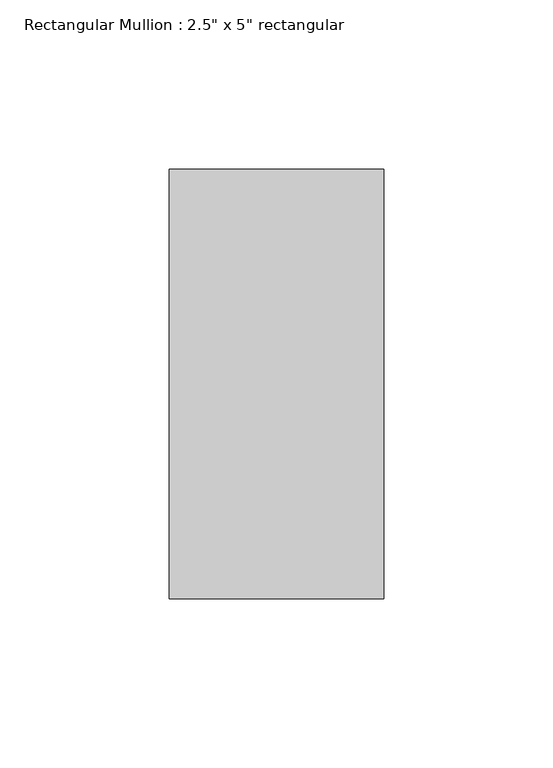
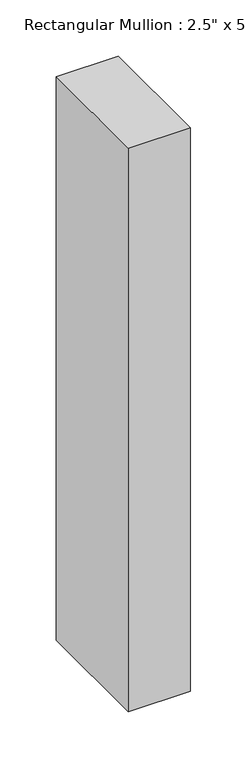
"""IFC4 building model written with IfcOpenShell, lengths in millimetres: member geometry."""

import ifcopenshell
import ifcopenshell.guid

model = None  # the IFC model being written
_history = None  # IfcOwnerHistory: only IFC2X3 demands one
_inside = {}  # id of a spatial element -> (the spatial element, [elements in it])
_under = {}  # id of a project, library or spatial element -> (it, [spatial elements below it])
_declared = {}  # id of a project -> (the project, [libraries it declares])
_typed = {}  # id of a type object -> (the type object, [elements of that type])
_made_of = {}  # id of a material, layer set ... -> (it, [elements and type objects made of it])


def new_model(schema):
    """Start an empty IFC model of exactly this schema.

    Asked for "IFC4X3", IfcOpenShell would pick the latest addendum, in which some entities
    have other attributes; the version numbers below select the first issue.
    IFC2X3 requires an IfcOwnerHistory on every rooted entity: one is made here for all.
    """
    global model, _history
    if schema == "IFC4X3":
        model = ifcopenshell.file(schema_version=(4, 3, 0, 0))
    else:
        model = ifcopenshell.file(schema=schema)
    _inside.clear()
    _under.clear()
    _declared.clear()
    _typed.clear()
    _made_of.clear()
    _history = None
    if model.schema == "IFC2X3":
        org = make("IfcOrganization", Name="unknown")
        user = make(
            "IfcPersonAndOrganization",
            ThePerson=make("IfcPerson", FamilyName="unknown"),
            TheOrganization=org,
        )
        app = make(
            "IfcApplication",
            ApplicationDeveloper=org,
            Version="unknown",
            ApplicationFullName="unknown",
            ApplicationIdentifier="unknown",
        )
        _history = make(
            "IfcOwnerHistory",
            OwningUser=user,
            OwningApplication=app,
            ChangeAction="ADDED",
            CreationDate=0,
        )
    return model


def make(cls, **values):
    """One entity of the class cls with the attributes given. An attribute that is None is left unset."""
    return model.create_entity(
        cls, **{name: value for name, value in values.items() if value is not None}
    )


def rooted(cls, **values):
    """An entity with a GlobalId (a new one), such as an element, a storey or a relation."""
    return make(cls, GlobalId=ifcopenshell.guid.new(), OwnerHistory=_history, **values)


def si_unit(unit_type, name, prefix=None):
    """IfcSIUnit, for example si_unit("LENGTHUNIT", "METRE", prefix="MILLI")."""
    return make("IfcSIUnit", UnitType=unit_type, Prefix=prefix, Name=name)


def assignment(units):
    """IfcUnitAssignment: the units of a project."""
    return None if units is None else make("IfcUnitAssignment", Units=units)


def point(xyz):
    """IfcCartesianPoint."""
    return None if xyz is None else make("IfcCartesianPoint", Coordinates=xyz)


def direction(xyz):
    """IfcDirection."""
    return None if xyz is None else make("IfcDirection", DirectionRatios=xyz)


def frame(location, z_axis=None, x_axis=None):
    """IfcAxis2Placement3D, a coordinate frame: its origin and axes. An axis left out is left unset."""
    return make(
        "IfcAxis2Placement3D",
        Location=point(location),
        Axis=direction(z_axis),
        RefDirection=direction(x_axis),
    )


def origin():
    """The frame at (0, 0, 0) with its axes left unset."""
    return frame((0.0, 0.0, 0.0))


def place(relative_to, where):
    """IfcLocalPlacement: puts the frame where relative to a parent placement (None: the world)."""
    return make(
        "IfcLocalPlacement", PlacementRelTo=relative_to, RelativePlacement=where
    )


def context(
    kind, dimensions, precision=None, world=None, true_north=None, identifier=None
):
    """IfcGeometricRepresentationContext, for example the 3D "Model" context."""
    return make(
        "IfcGeometricRepresentationContext",
        ContextIdentifier=identifier,
        ContextType=kind,
        CoordinateSpaceDimension=dimensions,
        Precision=precision,
        WorldCoordinateSystem=world,
        TrueNorth=true_north,
    )


def project(units=None, contexts=None):
    """IfcProject with its units and contexts."""
    return rooted(
        "IfcProject",
        Name="project",
        RepresentationContexts=contexts,
        UnitsInContext=assignment(units),
    )


def spatial(cls, under=None, at=None, **own):
    """A site, building, storey or space (cls), placed at a placement, below another one or the project."""
    s = rooted(cls, ObjectPlacement=at, **own)
    if under is not None:
        _under.setdefault(under.id(), (under, []))[1].append(s)
    return s


def polyline(points):
    """IfcPolyline through the points."""
    return make("IfcPolyline", Points=[point(p) for p in points])


def outline(outer, holes=None, kind="AREA"):
    """IfcArbitraryClosedProfileDef: a profile drawn as a closed curve; with holes, ...WithVoids."""
    if holes is None:
        return make("IfcArbitraryClosedProfileDef", ProfileType=kind, OuterCurve=outer)
    return make(
        "IfcArbitraryProfileDefWithVoids",
        ProfileType=kind,
        OuterCurve=outer,
        InnerCurves=holes,
    )


def extrude(swept, where, along, depth):
    """IfcExtrudedAreaSolid: the profile swept, set in the frame where, extruded along a direction by depth."""
    return make(
        "IfcExtrudedAreaSolid",
        SweptArea=swept,
        Position=where,
        ExtrudedDirection=direction(along),
        Depth=depth,
    )


def shape(context_of_items, identifier, shape_type, items):
    """IfcShapeRepresentation: the items that make up one representation, for example the "Body"."""
    return make(
        "IfcShapeRepresentation",
        ContextOfItems=context_of_items,
        RepresentationIdentifier=identifier,
        RepresentationType=shape_type,
        Items=items,
    )


def source(mapping_origin, context_of_items, identifier, shape_type, items):
    """IfcRepresentationMap: a shape defined once, which mapped items show again and again."""
    return make(
        "IfcRepresentationMap",
        MappingOrigin=mapping_origin,
        MappedRepresentation=shape(context_of_items, identifier, shape_type, items),
    )


def transform(
    local_origin,
    x_axis=None,
    y_axis=None,
    z_axis=None,
    scale=None,
    scale2=None,
    scale3=None,
    uniform=True,
):
    """IfcCartesianTransformationOperator3D, or its non-uniform kind. x_axis, y_axis, z_axis: its Axis1, 2, 3."""
    if uniform:
        return make(
            "IfcCartesianTransformationOperator3D",
            Axis1=direction(x_axis),
            Axis2=direction(y_axis),
            LocalOrigin=point(local_origin),
            Scale=scale,
            Axis3=direction(z_axis),
        )
    return make(
        "IfcCartesianTransformationOperator3DnonUniform",
        Axis1=direction(x_axis),
        Axis2=direction(y_axis),
        LocalOrigin=point(local_origin),
        Scale=scale,
        Axis3=direction(z_axis),
        Scale2=scale2,
        Scale3=scale3,
    )


def mapped(mapping_source, mapping_target):
    """IfcMappedItem: shows the shape of a source again, moved by a transform."""
    return make(
        "IfcMappedItem", MappingSource=mapping_source, MappingTarget=mapping_target
    )


def made_of(thing, what):
    """Note that an element or type object is made of a material, layer set ...; save() writes the relation."""
    if what is not None:
        _made_of.setdefault(what.id(), (what, []))[1].append(thing)
    return thing


def element(
    cls,
    number,
    at=None,
    inside=None,
    cuts=None,
    type_object=None,
    material=None,
    context=None,
    identifier="Body",
    shape_type=None,
    held_by="IfcProductDefinitionShape",
    body=None,
    shapes=None,
    **own,
):
    """One element of the class cls, such as IfcWall. Its Tag is "e" and its number.

    at: its placement. inside: the storey or other place that contains it. cuts: it is an
    opening in that element (IfcRelVoidsElement). A single representation is given by context,
    identifier, shape_type and body (its items); several are given by shapes. held_by: the class
    of the entity that holds the representations. save() writes the other relations.
    """
    e = rooted(cls, Tag="e%d" % number, ObjectPlacement=at, **own)
    if body is not None:
        shapes = [shape(context, identifier, shape_type, body)]
    if shapes is not None:
        e.Representation = make(held_by, Representations=shapes)
    if inside is not None:
        _inside.setdefault(inside.id(), (inside, []))[1].append(e)
    if cuts is not None:
        rooted(
            "IfcRelVoidsElement", RelatingBuildingElement=cuts, RelatedOpeningElement=e
        )
    if type_object is not None:
        _typed.setdefault(type_object.id(), (type_object, []))[1].append(e)
    return made_of(e, material)


def aggregate(whole, parts):
    """IfcRelAggregates: a whole, such as a stair, and the parts it consists of."""
    return rooted("IfcRelAggregates", RelatingObject=whole, RelatedObjects=parts)


def save(model, path):
    """Write the relations noted so far, then the file.

    IfcRelAggregates (storeys below a building ...), IfcRelContainedInSpatialStructure (elements
    in a storey), IfcRelDefinesByType, IfcRelAssociatesMaterial and IfcRelDeclares: one each for
    every whole, place, type object, material and project.
    """
    for whole, parts in _under.values():
        aggregate(whole, parts)
    for where, things in _inside.values():
        rooted(
            "IfcRelContainedInSpatialStructure",
            RelatedElements=things,
            RelatingStructure=where,
        )
    for kind, things in _typed.values():
        rooted("IfcRelDefinesByType", RelatedObjects=things, RelatingType=kind)
    for what, things in _made_of.values():
        rooted("IfcRelAssociatesMaterial", RelatedObjects=things, RelatingMaterial=what)
    for by, libraries in _declared.values():
        rooted("IfcRelDeclares", RelatingContext=by, RelatedDefinitions=libraries)
    model.write(path)


def member_6e77e263(model_context):
    return source(origin(), model_context, "Body", "SweptSolid", [
        extrude(outline(polyline([(31.75, 63.5), (31.75, -63.5), (-31.75, -63.5), (-31.75, 63.5), (31.75, 63.5)])), frame((0.0, 0.0, -609.6), z_axis=(0.0, 0.0, 1.0), x_axis=(1.0, 0.0, 0.0)), (0.0, 0.0, 1.0), 609.6),
    ])


if __name__ == "__main__":
    model = new_model("IFC4")
    model_context = context("Model", 3, world=origin())
    ifc_project = project(units=[si_unit("LENGTHUNIT", "METRE", prefix="MILLI")], contexts=[model_context])
    site = spatial("IfcSite", under=ifc_project)
    building = spatial("IfcBuilding", under=site)
    placement = place(None, origin())
    member_shape = member_6e77e263(model_context)
    element("IfcMember", 1, ObjectType="Rectangular Mullion : 2.5\" x 5\" rectangular", at=placement, inside=building, context=model_context, shape_type="MappedRepresentation", body=[
        mapped(member_shape, transform((0.0, 0.0, 0.0), x_axis=(1.0, 0.0, 0.0), y_axis=(0.0, 1.0, 0.0), z_axis=(0.0, 0.0, 1.0))),
    ])
    save(model, "model.ifc")

# Revit data of these elements
# Type "Rectangular Mullion : 2.5\" x 5\" rectangular"
#   built-in parameter 1007304 = 0.416667 (stored number, unit not read)
#   built-in parameter 1007301 = 0.104167 (stored number, unit not read)
#   built-in parameter 1007300 = 0.104167 (stored number, unit not read)
# Element 1 (IfcMember, "Rectangular Mullion : 2.5\" x 5\" rectangular")
#   Materials on its faces: "Aluminum"
# Materials
#   "Aluminum": class "Metal", colour RGB 247 247 247, transparency 0, Description = "Aluminum 6061", Cost = 0
